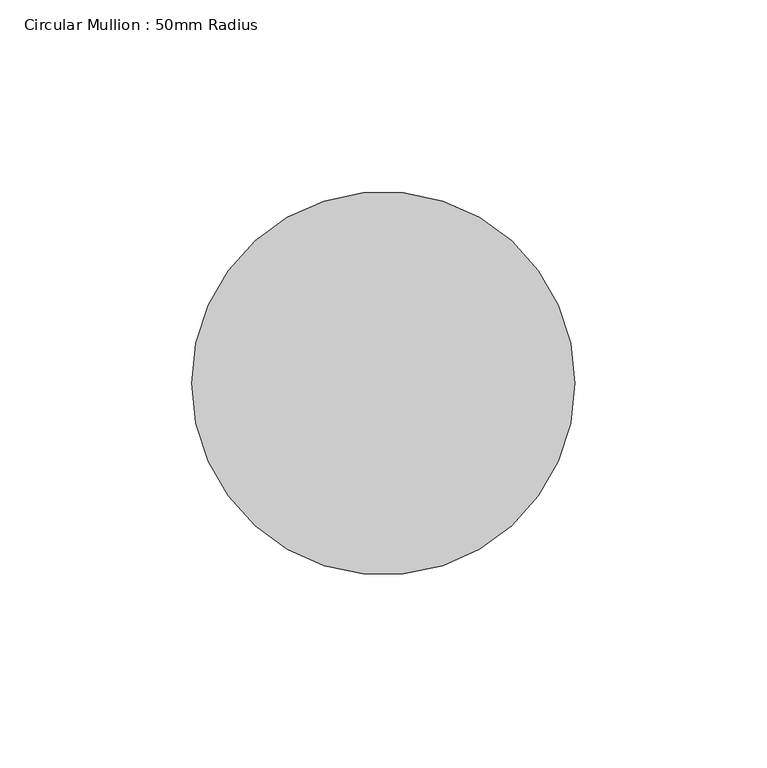
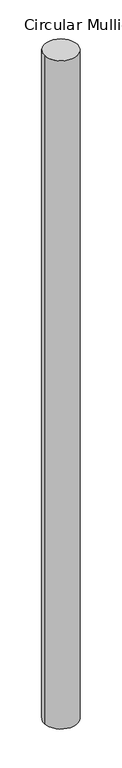
"""IFC4 building model written with IfcOpenShell, lengths in millimetres: member geometry, Circular Mullion : 50mm Radius."""

from ifc_helpers import new_model, si_unit, point, frame, origin, origin_2d, place, context, project, spatial, circle_curve, trimmed, segment, composite_curve, outline, extrude, source, transform, mapped, element, save


def circular_mullion_50mm_radius_b3b8e340(model_context):
    return source(origin(), model_context, "Body", "SweptSolid", [
        extrude(outline(composite_curve([segment(trimmed(circle_curve(origin_2d(), 50.0), [point((50.0, 0.0))], [point((-50.0, 0.0))], False, "CARTESIAN"), True, "CONTINUOUS"), segment(trimmed(circle_curve(origin_2d(), 50.0), [point((-50.0, 0.0))], [point((50.0, 0.0))], False, "CARTESIAN"), True, "CONTINUOUS")], self_intersect=False)), frame((0.0, 0.0, -2125.7270075), z_axis=(0.0, 0.0, 1.0), x_axis=(1.0, 0.0, 0.0)), (0.0, 0.0, 1.0), 2125.7270075),
    ])


if __name__ == "__main__":
    model = new_model("IFC4")
    model_context = context("Model", 3, world=origin())
    ifc_project = project(units=[si_unit("LENGTHUNIT", "METRE", prefix="MILLI")], contexts=[model_context])
    site = spatial("IfcSite", under=ifc_project)
    building = spatial("IfcBuilding", under=site)
    placement = place(None, origin())
    circular_mullion_50mm_radius_shape = circular_mullion_50mm_radius_b3b8e340(model_context)
    element("IfcMember", 1, ObjectType="Circular Mullion : 50mm Radius", at=placement, inside=building, context=model_context, shape_type="MappedRepresentation", body=[
        mapped(circular_mullion_50mm_radius_shape, transform((0.0, 0.0, 0.0), x_axis=(1.0, 0.0, 0.0), y_axis=(0.0, 1.0, 0.0), z_axis=(0.0, 0.0, 1.0))),
    ])
    save(model, "model.ifc")

# Revit data of these elements
# Type "Circular Mullion : 50mm Radius"
#   built-in parameter 1007350 = 0.164042 (stored number, unit not read)
# Element 1 (IfcMember, "Circular Mullion : 50mm Radius")
#   Materials on its faces: "Aluminium"
# Materials
#   "Aluminium": class "Metal", colour RGB 247 247 247, transparency 0, Description = "Aluminium 6061", Cost = 0
